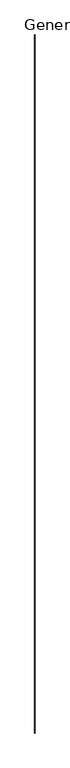
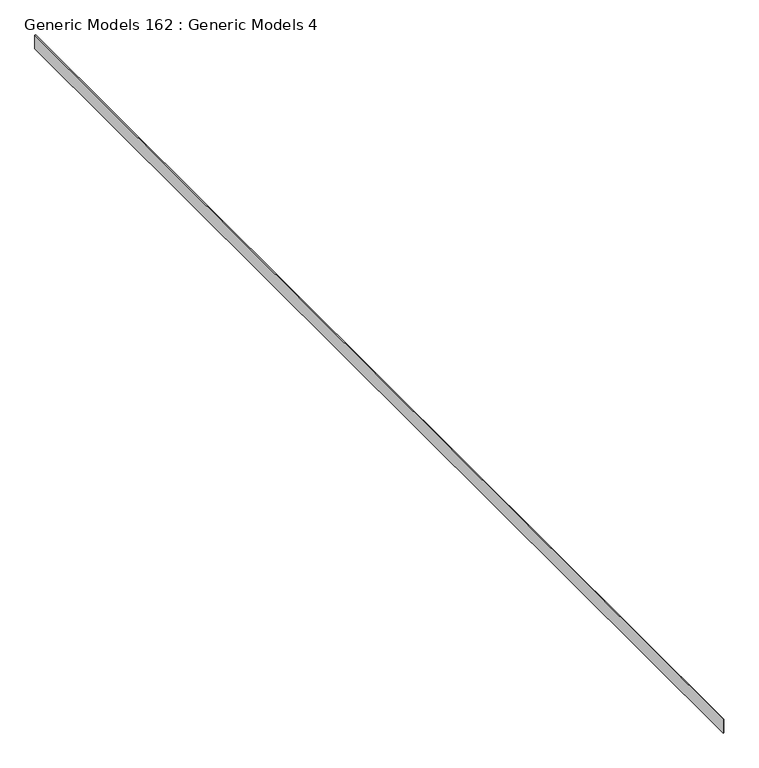
"""IFC4 building model written with IfcOpenShell, lengths in millimetres: proxy geometry, Generic Models 162 : Generic Models 4."""

from ifc_helpers import new_model, si_unit, origin, place, context, project, spatial, faceted_brep, source, transform, mapped, element, save


def generic_models_162_generic_models_4_6faf931f(model_context):
    return source(origin(), model_context, "Body", "Brep", [
        faceted_brep([(-10237.6972239, -5493.3230338, 122946.1234874), (-10237.6972239, -5493.3230338, 122897.0249647), (-10237.6972239, -5493.3230338, 122842.82201), (-10237.6972239, -5493.3230338, 122793.7234874), (-10231.3472239, -5493.3230338, 122793.7234874), (-10231.3472239, -5493.3230338, 122946.1234874), (-10237.6972239, 7054.2769662, 122946.1234874), (-10231.3472239, 7054.2769662, 122946.1234874), (-10231.3472239, 7054.2769662, 122793.7234874), (-10237.6972239, 7054.2769662, 122793.7234874), (-10237.6972239, 7054.2769662, 122842.82201), (-10237.6972239, 7054.2769662, 122897.0249648)], [[[0, 1, 2, 3, 4, 5]], [[6, 7, 8, 9, 10, 11]], [[3, 2, 1, 0, 6, 11, 10, 9]], [[4, 3, 9, 8]], [[5, 4, 8, 7]], [[0, 5, 7, 6]]]),
    ])


if __name__ == "__main__":
    model = new_model("IFC4")
    model_context = context("Model", 3, world=origin())
    ifc_project = project(units=[si_unit("LENGTHUNIT", "METRE", prefix="MILLI")], contexts=[model_context])
    site = spatial("IfcSite", under=ifc_project)
    building = spatial("IfcBuilding", under=site)
    placement = place(None, origin())
    generic_models_162_generic_models_4_shape = generic_models_162_generic_models_4_6faf931f(model_context)
    element("IfcBuildingElementProxy", 1, Name="Generic Models 162 : Generic Models 4", ObjectType="Generic Models 162 : Generic Models 4", at=placement, inside=building, context=model_context, shape_type="MappedRepresentation", body=[
        mapped(generic_models_162_generic_models_4_shape, transform((0.0, 0.0, 0.0), x_axis=(1.0, 0.0, 0.0), y_axis=(0.0, 1.0, 0.0), z_axis=(0.0, 0.0, 1.0))),
    ])
    save(model, "model.ifc")

# Revit data of these elements
# Element 1 (IfcBuildingElementProxy, "Generic Models 162 : Generic Models 4")
#   Materials on its faces: "_STEEL BASE PLATE AT EACH RAILING POST"
# Materials
#   "_STEEL BASE PLATE AT EACH RAILING POST": class "Generic", colour RGB 233 233 233, transparency 0, Cost = 0
